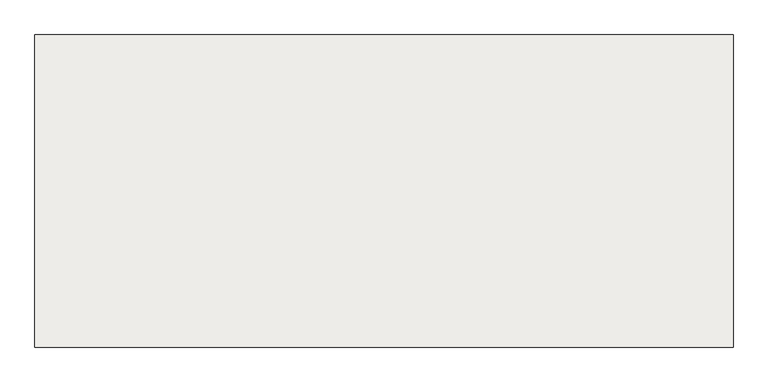
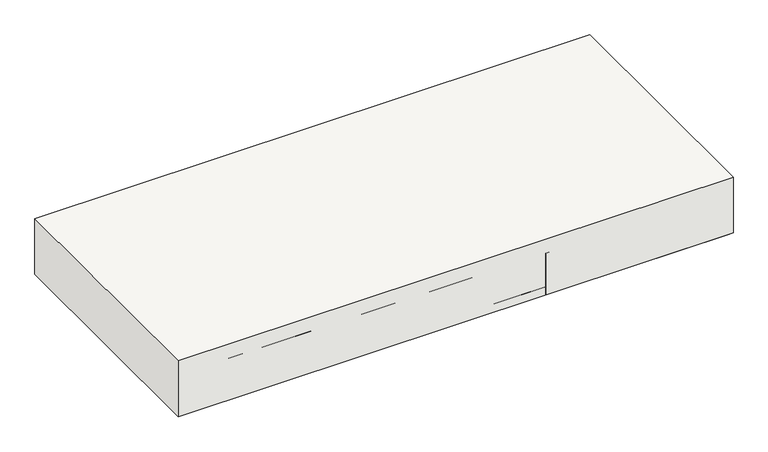
"""IFC4 building model written with IfcOpenShell, lengths in millimetres: slab geometry, Pano 19 (16 cm)."""

from ifc_helpers import new_model, si_unit, origin, origin_with_axes, place, context, project, spatial, polyline, outline, extrude, source, transform, mapped, element, save


def slab_c5574e0f(model_context):
    return source(origin(), model_context, "Body", "SweptSolid", [
        extrude(outline(polyline([(4250.0, 3685.0), (4250.0, 4360.0), (5760.0, 4360.0), (5760.0, 3685.0), (4250.0, 3685.0)])), origin_with_axes(), (0.0, 0.0, 1.0), 160.0),
        extrude(outline(polyline([(4750.0, 3685.0), (4610.0, 3685.0), (4610.0, 4360.0), (4750.0, 4360.0), (4750.0, 3685.0)])), origin_with_axes(), (0.0, 0.0, 1.0), 24.0),
        extrude(outline(polyline([(5110.0, 4185.0), (4750.0, 4185.0), (4750.0, 4355.0), (5110.0, 4355.0), (5110.0, 4185.0)])), origin_with_axes(), (0.0, 0.0, 1.0), 120.0),
        extrude(outline(polyline([(5610.0, 3685.0), (5250.0, 3685.0), (5250.0, 4180.0), (5610.0, 4180.0), (5610.0, 3685.0)])), origin_with_axes(), (0.0, 0.0, 1.0), 120.0),
        extrude(outline(polyline([(5750.0, 3685.0), (5610.0, 3685.0), (5610.0, 4360.0), (5750.0, 4360.0), (5750.0, 3685.0)])), origin_with_axes(), (0.0, 0.0, 1.0), 24.0),
        extrude(outline(polyline([(4610.5, 4185.0), (4250.5, 4185.0), (4250.5, 4355.0), (4610.5, 4355.0), (4610.5, 4185.0)])), origin_with_axes(), (0.0, 0.0, 1.0), 120.0),
        extrude(outline(polyline([(5250.0, 3685.0), (5110.0, 3685.0), (5110.0, 4360.0), (5250.0, 4360.0), (5250.0, 3685.0)])), origin_with_axes(), (0.0, 0.0, 1.0), 24.0),
        extrude(outline(polyline([(5610.0, 4185.0), (5250.0, 4185.0), (5250.0, 4355.0), (5610.0, 4355.0), (5610.0, 4185.0)])), origin_with_axes(), (0.0, 0.0, 1.0), 120.0),
        extrude(outline(polyline([(4610.5, 3685.0), (4250.5, 3685.0), (4250.5, 4180.0), (4610.5, 4180.0), (4610.5, 3685.0)])), origin_with_axes(), (0.0, 0.0, 1.0), 120.0),
        extrude(outline(polyline([(5110.0, 3685.0), (4750.0, 3685.0), (4750.0, 4180.0), (5110.0, 4180.0), (5110.0, 3685.0)])), origin_with_axes(), (0.0, 0.0, 1.0), 120.0),
    ])


if __name__ == "__main__":
    model = new_model("IFC4")
    model_context = context("Model", 3, world=origin())
    ifc_project = project(units=[si_unit("LENGTHUNIT", "METRE", prefix="MILLI")], contexts=[model_context])
    site = spatial("IfcSite", under=ifc_project)
    building = spatial("IfcBuilding", under=site)
    placement = place(None, origin())
    slab_shape = slab_c5574e0f(model_context)
    element("IfcSlab", 1, ObjectType="Pano 19 (16 cm)", at=placement, inside=building, context=model_context, shape_type="MappedRepresentation", body=[
        mapped(slab_shape, transform((0.0, 0.0, 0.0), x_axis=(1.0, 0.0, 0.0), y_axis=(0.0, 1.0, 0.0), z_axis=(0.0, 0.0, 1.0))),
    ])
    save(model, "model.ifc")

# Revit data of these elements
# Element 1 (IfcSlab, "Pano 19 (16 cm)")
#   Materials on its faces: "Molde de poliestireno", "Concreto armado", "RGB 168-169-158"
# Materials
#   "Molde de poliestireno": class "Não atribuído", colour RGB 255 255 255, transparency 0
#   "Concreto armado": class "Não atribuído", colour RGB 168 169 158, transparency 0
#   "RGB 168-169-158": class "Não atribuído", colour RGB 168 169 158, transparency 0
